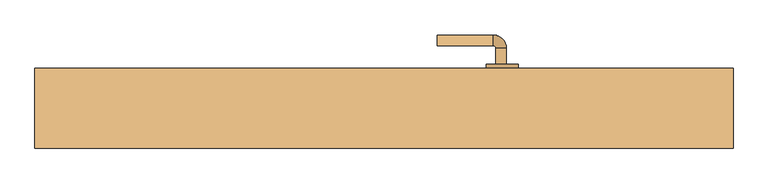
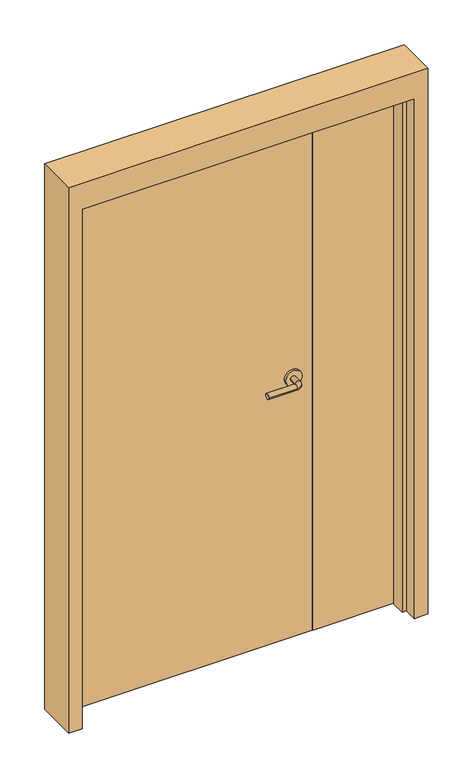
"""IFC4 building model written with IfcOpenShell, lengths in millimetres: door geometry, Дверь-Маятниковая-С полотнами разной ширины-Щитовая : 1310 x 2100 мм."""

from ifc_helpers import new_model, si_unit, point, frame, frame_2d, origin, origin_with_axes, place, context, project, spatial, polyline, circle_curve, ellipse_curve, trimmed, segment, composite_curve, outline, extrude, faceted_brep, source, transform, mapped, element, save
from ifc_brep_helpers import plane_surface, cylinder_surface, revolved_surface, advanced_brep


def door_0ca85bf1(model_context):
    return source(origin(), model_context, "Body", "SolidModel", [
        advanced_brep(
        [(229.59375, -9.15, 1000.0), (209.59375, -9.15, 1000.0), (229.59375, -39.15, 1000.0), (209.59375, -39.15, 1000.0), (204.59375, -44.15, 1000.0), (204.59375, -64.15, 1000.0), (99.59375, -64.15, 1000.0), (99.59375, -44.15, 1000.0)],
        [
            (0, 1, circle_curve(frame((219.59375, -9.15, 1000.0), z_axis=(0.0, 1.0, 0.0), x_axis=(-1.0, 0.0, 0.0)), 10.0)),
            (1, 0, circle_curve(frame((219.59375, -9.15, 1000.0), z_axis=(0.0, 1.0, 0.0), x_axis=(-1.0, 0.0, 0.0)), 10.0)),
            (0, 2),
            (2, 3, circle_curve(frame((219.59375, -39.15, 1000.0), z_axis=(0.0, 1.0, 0.0), x_axis=(-1.0, 0.0, 0.0)), 10.0)),
            (3, 1),
            (3, 2, circle_curve(frame((219.59375, -39.15, 1000.0), z_axis=(0.0, 1.0, 0.0), x_axis=(-1.0, 0.0, 0.0)), 10.0)),
            (4, 3, circle_curve(frame((204.59375, -39.15, 1000.0), z_axis=(0.0, 0.0, 1.0), x_axis=(1.0, 0.0, 0.0)), 5.0)),
            (2, 5, circle_curve(frame((204.59375, -39.15, 1000.0), z_axis=(0.0, 0.0, -1.0), x_axis=(1.0, 0.0, 0.0)), 25.0)),
            (5, 4, circle_curve(frame((204.59375, -54.15, 1000.0), z_axis=(1.0, 0.0, 0.0), x_axis=(0.0, 1.0, 0.0)), 10.0)),
            (4, 5, circle_curve(frame((204.59375, -54.15, 1000.0), z_axis=(1.0, 0.0, 0.0), x_axis=(0.0, 1.0, 0.0)), 10.0)),
            (6, 7, circle_curve(frame((99.59375, -54.15, 1000.0), z_axis=(-1.0, 0.0, 0.0), x_axis=(0.0, 1.0, 0.0)), 10.0)),
            (7, 6, circle_curve(frame((99.59375, -54.15, 1000.0), z_axis=(-1.0, 0.0, 0.0), x_axis=(0.0, 1.0, 0.0)), 10.0)),
            (5, 6),
            (7, 4),
        ],
        [
            plane_surface(frame((219.59375, -9.15, 1000.0), z_axis=(0.0, 1.0, 0.0), x_axis=(0.0, 0.0, 1.0))),
            cylinder_surface(frame((219.59375, -9.15, 1000.0), z_axis=(0.0, 1.0, 0.0), x_axis=(-1.0, 0.0, 0.0)), 10.0),
            revolved_surface(trimmed(ellipse_curve(frame((219.59375, -39.15, 1000.0), z_axis=(0.0, 1.0, 0.0), x_axis=(-1.0, 0.0, 0.0)), 10.0, 10.0), [point((229.59375, -39.15, 1000.0))], [point((209.59375, -39.15, 1000.0))], True, "CARTESIAN"), (204.59375, -39.15, 1000.0), (0.0, 0.0, -1.0)),
            revolved_surface(trimmed(ellipse_curve(frame((219.59375, -39.15, 1000.0), z_axis=(0.0, 1.0, 0.0), x_axis=(-1.0, 0.0, 0.0)), 10.0, 10.0), [point((209.59375, -39.15, 1000.0))], [point((229.59375, -39.15, 1000.0))], True, "CARTESIAN"), (204.59375, -39.15, 1000.0), (0.0, 0.0, -1.0)),
            plane_surface(frame((99.59375, -54.15, 1000.0), z_axis=(-1.0, 0.0, 0.0), x_axis=(0.0, 0.0, 1.0))),
            cylinder_surface(frame((204.59375, -54.15, 1000.0), z_axis=(1.0, 0.0, 0.0), x_axis=(0.0, 1.0, 0.0)), 10.0),
        ],
        [
            (0, [[1, 2]]),
            (1, [[-1, 3, 4, 5]]),
            (1, [[-2, -5, 6, -3]]),
            (2, [[7, -4, 8, 9]]),
            (3, [[-8, -6, -7, 10]]),
            (4, [[11, 12]]),
            (5, [[-9, 13, -12, 14]]),
            (5, [[-10, -14, -11, -13]]),
        ],
    ),
        extrude(outline(composite_curve([segment(trimmed(circle_curve(frame_2d((1000.0, 222.09375)), 30.0), [point((1000.0, 252.09375))], [point((1000.0, 192.09375))], False, "CARTESIAN"), True, "CONTINUOUS"), segment(trimmed(circle_curve(frame_2d((1000.0, 222.09375)), 30.0), [point((1000.0, 192.09375))], [point((1000.0, 252.09375))], False, "CARTESIAN"), True, "CONTINUOUS")], self_intersect=False)), frame((0.0, -9.15, 0.0), z_axis=(0.0, 1.0, 0.0), x_axis=(0.0, 0.0, 1.0)), (0.0, 0.0, 1.0), 8.0),
        advanced_brep(
        [(229.59375, 51.85, 1000.0), (209.59375, 51.85, 1000.0), (209.59375, 81.85, 1000.0), (229.59375, 81.85, 1000.0), (204.59375, 86.85, 1000.0), (204.59375, 106.85, 1000.0), (99.59375, 106.85, 1000.0), (99.59375, 86.85, 1000.0)],
        [
            (0, 1, circle_curve(frame((219.59375, 51.85, 1000.0), z_axis=(0.0, -1.0, 0.0), x_axis=(-1.0, 0.0, 0.0)), 10.0)),
            (1, 0, circle_curve(frame((219.59375, 51.85, 1000.0), z_axis=(0.0, -1.0, 0.0), x_axis=(-1.0, 0.0, 0.0)), 10.0)),
            (1, 2),
            (2, 3, circle_curve(frame((219.59375, 81.85, 1000.0), z_axis=(0.0, -1.0, 0.0), x_axis=(-1.0, 0.0, 0.0)), 10.0)),
            (3, 0),
            (3, 2, circle_curve(frame((219.59375, 81.85, 1000.0), z_axis=(0.0, -1.0, 0.0), x_axis=(-1.0, 0.0, 0.0)), 10.0)),
            (4, 5, circle_curve(frame((204.59375, 96.85, 1000.0), z_axis=(1.0, 0.0, 0.0), x_axis=(0.0, -1.0, 0.0)), 10.0)),
            (5, 3, circle_curve(frame((204.59375, 81.85, 1000.0), z_axis=(0.0, 0.0, -1.0), x_axis=(1.0, 0.0, 0.0)), 25.0)),
            (2, 4, circle_curve(frame((204.59375, 81.85, 1000.0), z_axis=(0.0, 0.0, 1.0), x_axis=(1.0, 0.0, 0.0)), 5.0)),
            (5, 4, circle_curve(frame((204.59375, 96.85, 1000.0), z_axis=(1.0, 0.0, 0.0), x_axis=(0.0, -1.0, 0.0)), 10.0)),
            (6, 7, circle_curve(frame((99.59375, 96.85, 1000.0), z_axis=(-1.0, 0.0, 0.0), x_axis=(0.0, -1.0, 0.0)), 10.0)),
            (7, 6, circle_curve(frame((99.59375, 96.85, 1000.0), z_axis=(-1.0, 0.0, 0.0), x_axis=(0.0, -1.0, 0.0)), 10.0)),
            (4, 7),
            (6, 5),
        ],
        [
            plane_surface(frame((219.59375, 51.85, 1000.0), z_axis=(0.0, -1.0, 0.0), x_axis=(0.0, 0.0, 1.0))),
            cylinder_surface(frame((219.59375, 51.85, 1000.0), z_axis=(0.0, -1.0, 0.0), x_axis=(-1.0, 0.0, 0.0)), 10.0),
            revolved_surface(trimmed(ellipse_curve(frame((219.59375, 81.85, 1000.0), z_axis=(0.0, 1.0, 0.0), x_axis=(-1.0, 0.0, 0.0)), 10.0, 10.0), [point((229.59375, 81.85, 1000.0))], [point((209.59375, 81.85, 1000.0))], True, "CARTESIAN"), (204.59375, 81.85, 1000.0), (0.0, 0.0, -1.0)),
            revolved_surface(trimmed(ellipse_curve(frame((219.59375, 81.85, 1000.0), z_axis=(0.0, 1.0, 0.0), x_axis=(-1.0, 0.0, 0.0)), 10.0, 10.0), [point((209.59375, 81.85, 1000.0))], [point((229.59375, 81.85, 1000.0))], True, "CARTESIAN"), (204.59375, 81.85, 1000.0), (0.0, 0.0, -1.0)),
            plane_surface(frame((99.59375, 96.85, 1000.0), z_axis=(-1.0, 0.0, 0.0), x_axis=(0.0, 0.0, 1.0))),
            cylinder_surface(frame((204.59375, 96.85, 1000.0), z_axis=(1.0, 0.0, 0.0), x_axis=(0.0, -1.0, 0.0)), 10.0),
        ],
        [
            (0, [[1, 2]]),
            (1, [[3, 4, 5, -2]]),
            (1, [[-5, 6, -3, -1]]),
            (2, [[7, 8, -4, 9]]),
            (3, [[10, -9, -6, -8]]),
            (4, [[11, 12]]),
            (5, [[13, -11, 14, -7]]),
            (5, [[-14, -12, -13, -10]]),
        ],
    ),
        extrude(outline(composite_curve([segment(trimmed(circle_curve(frame_2d((1000.0, 222.09375)), 30.0), [point((1000.0, 252.09375))], [point((1000.0, 192.09375))], False, "CARTESIAN"), True, "CONTINUOUS"), segment(trimmed(circle_curve(frame_2d((1000.0, 222.09375)), 30.0), [point((1000.0, 192.09375))], [point((1000.0, 252.09375))], False, "CARTESIAN"), True, "CONTINUOUS")], self_intersect=False)), frame((0.0, 43.85, 0.0), z_axis=(0.0, 1.0, 0.0), x_axis=(0.0, 0.0, 1.0)), (0.0, 0.0, 1.0), 8.0),
        extrude(outline(polyline([(605.0, -1.15), (296.6, -1.15), (296.6, 43.85), (605.0, 43.85), (605.0, -1.15)])), origin_with_axes(), (0.0, 0.0, 1.0), 2000.0),
        faceted_brep([(605.0, -5.9125, 0.0), (605.0, 43.85, 0.0), (655.0, 43.85, 0.0), (655.0, -106.15, 0.0), (605.0, -106.15, 0.0), (605.0, -56.9375, 0.0), (589.125, -56.9375, 0.0), (589.125, -5.9125, 0.0), (605.0, -5.9125, 2000.0), (605.0, 43.85, 2000.0), (-605.0, 43.85, 2000.0), (-605.0, 43.85, 0.0), (-655.0, 43.85, 0.0), (-655.0, 43.85, 2100.0), (655.0, 43.85, 2100.0), (655.0, -106.15, 2100.0), (-655.0, -106.15, 2100.0), (-655.0, -106.15, 0.0), (-605.0, -106.15, 0.0), (-605.0, -106.15, 2000.0), (605.0, -106.15, 2000.0), (605.0, -56.9375, 2000.0), (-605.0, -56.9375, 2000.0), (-605.0, -56.9375, 0.0), (-589.125, -56.9375, 0.0), (-589.125, -56.9375, 1984.125), (589.125, -56.9375, 1984.125), (589.125, -5.9125, 1984.125), (-589.125, -5.9125, 1984.125), (-589.125, -5.9125, 0.0), (-605.0, -5.9125, 0.0), (-605.0, -5.9125, 2000.0)], [[[0, 1, 2, 3, 4, 5, 6, 7]], [[1, 0, 8, 9]], [[2, 1, 9, 10, 11, 12, 13, 14]], [[3, 2, 14, 15]], [[4, 3, 15, 16, 17, 18, 19, 20]], [[5, 4, 20, 21]], [[6, 5, 21, 22, 23, 24, 25, 26]], [[7, 6, 26, 27]], [[0, 7, 27, 28, 29, 30, 31, 8]], [[9, 8, 31, 10]], [[20, 19, 22, 21]], [[26, 25, 28, 27]], [[12, 11, 30, 29, 24, 23, 18, 17]], [[11, 10, 31, 30]], [[13, 12, 17, 16]], [[19, 18, 23, 22]], [[25, 24, 29, 28]], [[15, 14, 13, 16]]]),
        extrude(outline(polyline([(293.4, -1.15), (-605.0, -1.15), (-605.0, 43.85), (293.4, 43.85), (293.4, -1.15)])), origin_with_axes(), (0.0, 0.0, 1.0), 2000.0),
    ])


if __name__ == "__main__":
    model = new_model("IFC4")
    model_context = context("Model", 3, world=origin())
    ifc_project = project(units=[si_unit("LENGTHUNIT", "METRE", prefix="MILLI")], contexts=[model_context])
    site = spatial("IfcSite", under=ifc_project)
    building = spatial("IfcBuilding", under=site)
    placement = place(None, origin())
    door_shape = door_0ca85bf1(model_context)
    element("IfcDoor", 1, ObjectType="Дверь-Маятниковая-С полотнами разной ширины-Щитовая : 1310 x 2100 мм", at=placement, inside=building, context=model_context, shape_type="MappedRepresentation", body=[
        mapped(door_shape, transform((0.0, 0.0, 0.0), x_axis=(1.0, 0.0, 0.0), y_axis=(0.0, 1.0, 0.0), z_axis=(0.0, 0.0, 1.0))),
    ])
    save(model, "model.ifc")

# Revit data of these elements
# Project information
#   Наименование здания = "Наименование здания"
#   Разработчики шаблона = "http://bim2b.ru"
#   Версия шаблона = "1.0.2"
#   Дата утверждения проекта = "Дата"
#   Статус проекта = "П"
#   Заказчик = "Заказчик"
#   Адрес проекта = "Адрес проекта"
#   Наименование проекта = "Наименование проекта"
#   Номер проекта = "Номер проекта"
#   RoomBookInternationalBuildNumber = "ZgA=BAAAAA==2018BgFlAAAAAQQAAAABAQAAAAYBZAAAAAHiBwAABAQAAAABTwQAAAcH1"
# Type "Дверь-Маятниковая-С полотнами разной ширины-Щитовая : 1310 x 2100 мм"
#   Type Mark = "150"
#   Assembly Code = "C1020300"
#   Analytic Construction = "Деревянный"
#   Ширина большой панели = 900 mm
#   W = 310 mm
#   Thickness = 45 mm
#   Thermal Resistance (R) = 0.455703 (m²·K)/W
#   Угол поворота [instance default] = 90°
#   Высота планки = 1000 mm
#   Rough Width [instance default] = 1310 mm
#   Rough Height [instance default] = 2100 mm
#   Высота проема в кирпичном каркасе [instance default] = 100 mm
#   Ширина проема в кирпичном каркасе [instance default] = 100 mm
#   Расчет вставки [instance default] = 105 mm
#   Кирпичная вставка [instance default] = 25 mm
#   Height = 2000 mm
#   Width = 1210 mm
#   Heat Transfer Coefficient (U) = 2.19465 W/(m²·K)
#   Глубина кирпичного каркаса = 150 mm
#   Кирпичный каркас [instance default] = yes
#   Каркас стены сухой кладки [instance default] = no
#   Материал панели = Древесина - Береза
#   Материал каркаса = Металл - Окрашенный - Серый 2
#   Материал дверной ручки = Алюминий
#   Visual Light Transmittance = 0
#   Solar Heat Gain Coefficient = 0
#   Wall Closure = (empty or 0)
#   Function = (empty or 0)
# Element 1 (IfcDoor, "Дверь-Маятниковая-С полотнами разной ширины-Щитовая : 1310 x 2100 мм")
#   Materials on its faces: "Алюминий", "Металл - Окрашенный - Серый 2", "Древесина - Береза"
# Materials
#   "Древесина - Береза": class "Древесина", colour RGB 166 116 52, transparency 0, Cost = 0
#   "Металл - Окрашенный - Серый 2": class "Краска", colour RGB 104 104 104, transparency 0, Cost = 0
#   "Алюминий": class "Металл", colour RGB 247 247 247, transparency 0
